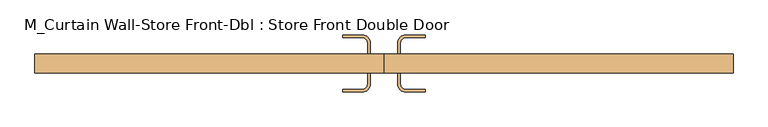
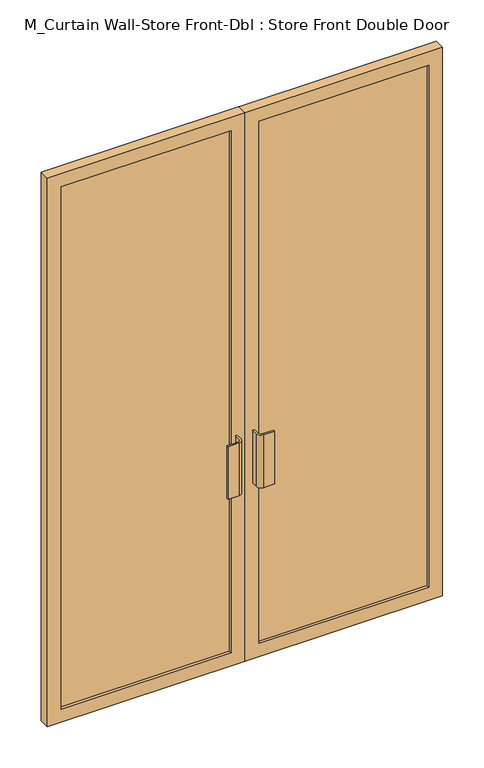
"""IFC4 building model written with IfcOpenShell, lengths in millimetres: door geometry, M_Curtain Wall-Store Front-Dbl : Store Front Double Door."""

from ifc_helpers import new_model, si_unit, point, frame, frame_2d, origin, place, context, project, spatial, polyline, circle_curve, trimmed, segment, composite_curve, outline, extrude, source, transform, mapped, element, save


def m_curtain_wall_store_front_dbl_store_front_double_door_f57a5871(model_context):
    return source(origin(), model_context, "Body", "SweptSolid", [
        extrude(outline(composite_curve([segment(trimmed(circle_curve(frame_2d((-50.8, -14.85)), 19.05), [point((-31.75, -14.85))], [point((-50.8, -33.9))], False, "CARTESIAN"), True, "CONTINUOUS"), segment(polyline([(-50.8, -33.9), (-95.25, -33.9), (-95.25, -27.55), (-50.8, -27.55)]), True, "CONTINUOUS"), segment(trimmed(circle_curve(frame_2d((-50.8, -14.85)), 12.7), [point((-50.8, -27.55))], [point((-38.1, -14.85))], True, "CARTESIAN"), True, "CONTINUOUS"), segment(polyline([(-38.1, -14.85), (-38.1, 10.55), (-31.75, 10.55), (-31.75, -14.85)]), True, "CONTINUOUS")], self_intersect=False)), frame((0.0, 0.0, 762.0), z_axis=(0.0, 0.0, 1.0), x_axis=(1.0, 0.0, 0.0)), (0.0, 0.0, 1.0), 228.6),
        extrude(outline(composite_curve([segment(polyline([(31.75, -14.85), (31.75, 10.55), (38.1, 10.55), (38.1, -14.85)]), True, "CONTINUOUS"), segment(trimmed(circle_curve(frame_2d((50.8, -14.85)), 12.7), [point((38.1, -14.85))], [point((50.8, -27.55))], True, "CARTESIAN"), True, "CONTINUOUS"), segment(polyline([(50.8, -27.55), (95.25, -27.55), (95.25, -33.9), (50.8, -33.9)]), True, "CONTINUOUS"), segment(trimmed(circle_curve(frame_2d((50.8, -14.85)), 19.05), [point((50.8, -33.9))], [point((31.75, -14.85))], False, "CARTESIAN"), True, "CONTINUOUS")], self_intersect=False)), frame((0.0, 0.0, 762.0), z_axis=(0.0, 0.0, 1.0), x_axis=(1.0, 0.0, 0.0)), (0.0, 0.0, 1.0), 228.6),
        extrude(outline(composite_curve([segment(polyline([(-31.75, 80.4), (-31.75, 55.0), (-38.1, 55.0), (-38.1, 80.4)]), True, "CONTINUOUS"), segment(trimmed(circle_curve(frame_2d((-50.8, 80.4)), 12.7), [point((-38.1, 80.4))], [point((-50.8, 93.1))], True, "CARTESIAN"), True, "CONTINUOUS"), segment(polyline([(-50.8, 93.1), (-95.25, 93.1), (-95.25, 99.45), (-50.8, 99.45)]), True, "CONTINUOUS"), segment(trimmed(circle_curve(frame_2d((-50.8, 80.4)), 19.05), [point((-50.8, 99.45))], [point((-31.75, 80.4))], False, "CARTESIAN"), True, "CONTINUOUS")], self_intersect=False)), frame((0.0, 0.0, 762.0), z_axis=(0.0, 0.0, 1.0), x_axis=(1.0, 0.0, 0.0)), (0.0, 0.0, 1.0), 228.6),
        extrude(outline(composite_curve([segment(trimmed(circle_curve(frame_2d((50.8, 80.4)), 19.05), [point((31.75, 80.4))], [point((50.8, 99.45))], False, "CARTESIAN"), True, "CONTINUOUS"), segment(polyline([(50.8, 99.45), (95.25, 99.45), (95.25, 93.1), (50.8, 93.1)]), True, "CONTINUOUS"), segment(trimmed(circle_curve(frame_2d((50.8, 80.4)), 12.7), [point((50.8, 93.1))], [point((38.1, 80.4))], True, "CARTESIAN"), True, "CONTINUOUS"), segment(polyline([(38.1, 80.4), (38.1, 55.0), (31.75, 55.0), (31.75, 80.4)]), True, "CONTINUOUS")], self_intersect=False)), frame((0.0, 0.0, 762.0), z_axis=(0.0, 0.0, 1.0), x_axis=(1.0, 0.0, 0.0)), (0.0, 0.0, 1.0), 228.6),
        extrude(outline(polyline([(752.85, 23.25), (57.94375, 23.25), (57.94375, 42.3), (752.85, 42.3), (752.85, 23.25)])), frame((0.0, 0.0, 57.15), z_axis=(0.0, 0.0, 1.0), x_axis=(1.0, 0.0, 0.0)), (0.0, 0.0, 1.0), 2260.7),
        extrude(outline(polyline([(-57.94375, 23.25), (-752.85, 23.25), (-752.85, 42.3), (-57.94375, 42.3), (-57.94375, 23.25)])), frame((0.0, 0.0, 57.15), z_axis=(0.0, 0.0, 1.0), x_axis=(1.0, 0.0, 0.0)), (0.0, 0.0, 1.0), 2260.7),
        extrude(outline(polyline([(2375.0, 0.79375), (0.0, 0.79375), (0.0, 810.0), (2375.0, 810.0), (2375.0, 0.79375)]), holes=[polyline([(2317.85, 57.94375), (2317.85, 752.85), (57.15, 752.85), (57.15, 57.94375), (2317.85, 57.94375)])]), frame((0.0, 10.55, 0.0), z_axis=(0.0, 1.0, 0.0), x_axis=(0.0, 0.0, 1.0)), (0.0, 0.0, 1.0), 44.45),
        extrude(outline(polyline([(2375.0, -0.79375), (2375.0, -810.0), (0.0, -810.0), (0.0, -0.79375), (2375.0, -0.79375)]), holes=[polyline([(2317.85, -752.85), (2317.85, -57.94375), (57.15, -57.94375), (57.15, -752.85), (2317.85, -752.85)])]), frame((0.0, 10.55, 0.0), z_axis=(0.0, 1.0, 0.0), x_axis=(0.0, 0.0, 1.0)), (0.0, 0.0, 1.0), 44.45),
    ])


if __name__ == "__main__":
    model = new_model("IFC4")
    model_context = context("Model", 3, world=origin())
    ifc_project = project(units=[si_unit("LENGTHUNIT", "METRE", prefix="MILLI")], contexts=[model_context])
    site = spatial("IfcSite", under=ifc_project)
    building = spatial("IfcBuilding", under=site)
    placement = place(None, origin())
    m_curtain_wall_store_front_dbl_store_front_double_door_shape = m_curtain_wall_store_front_dbl_store_front_double_door_f57a5871(model_context)
    element("IfcDoor", 1, ObjectType="M_Curtain Wall-Store Front-Dbl : Store Front Double Door", at=placement, inside=building, context=model_context, shape_type="MappedRepresentation", body=[
        mapped(m_curtain_wall_store_front_dbl_store_front_double_door_shape, transform((0.0, 0.0, 0.0), x_axis=(1.0, 0.0, 0.0), y_axis=(0.0, 1.0, 0.0), z_axis=(0.0, 0.0, 1.0))),
    ])
    save(model, "model.ifc")

# Revit data of these elements
# Type "M_Curtain Wall-Store Front-Dbl : Store Front Double Door"
#   Type Mark = "33"
#   Offset = 55 mm
#   Function = 1
#   Material = Metal - Aluminum
#   Glazing Material = Glass
#   Assembly Code = ""
# Element 1 (IfcDoor, "M_Curtain Wall-Store Front-Dbl : Store Front Double Door")
#   Materials on its faces: "Metal - Aluminum", "Glass"
# Materials
#   "Metal - Aluminum": class "Metal", colour RGB 247 247 247, transparency 0
#   "Glass": class "Glass", colour RGB 0 128 192, transparency 0.9
